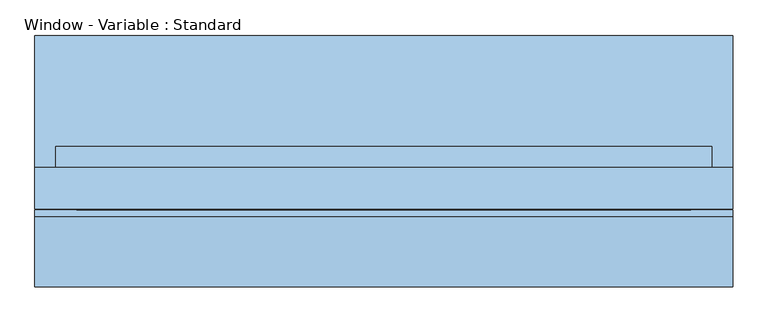
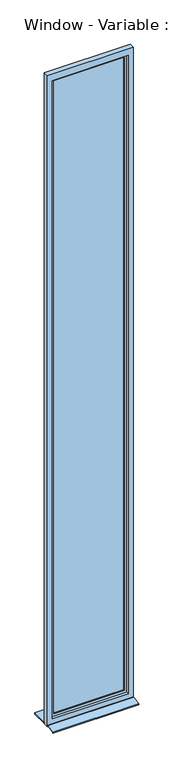
"""IFC4 building model written with IfcOpenShell, lengths in millimetres: window geometry, Window - Variable : Standard."""

import ifcopenshell
import ifcopenshell.guid

model = None  # the IFC model being written
_history = None  # IfcOwnerHistory: only IFC2X3 demands one
_inside = {}  # id of a spatial element -> (the spatial element, [elements in it])
_under = {}  # id of a project, library or spatial element -> (it, [spatial elements below it])
_declared = {}  # id of a project -> (the project, [libraries it declares])
_typed = {}  # id of a type object -> (the type object, [elements of that type])
_made_of = {}  # id of a material, layer set ... -> (it, [elements and type objects made of it])


def new_model(schema):
    """Start an empty IFC model of exactly this schema.

    Asked for "IFC4X3", IfcOpenShell would pick the latest addendum, in which some entities
    have other attributes; the version numbers below select the first issue.
    IFC2X3 requires an IfcOwnerHistory on every rooted entity: one is made here for all.
    """
    global model, _history
    if schema == "IFC4X3":
        model = ifcopenshell.file(schema_version=(4, 3, 0, 0))
    else:
        model = ifcopenshell.file(schema=schema)
    _inside.clear()
    _under.clear()
    _declared.clear()
    _typed.clear()
    _made_of.clear()
    _history = None
    if model.schema == "IFC2X3":
        org = make("IfcOrganization", Name="unknown")
        user = make(
            "IfcPersonAndOrganization",
            ThePerson=make("IfcPerson", FamilyName="unknown"),
            TheOrganization=org,
        )
        app = make(
            "IfcApplication",
            ApplicationDeveloper=org,
            Version="unknown",
            ApplicationFullName="unknown",
            ApplicationIdentifier="unknown",
        )
        _history = make(
            "IfcOwnerHistory",
            OwningUser=user,
            OwningApplication=app,
            ChangeAction="ADDED",
            CreationDate=0,
        )
    return model


def make(cls, **values):
    """One entity of the class cls with the attributes given. An attribute that is None is left unset."""
    return model.create_entity(
        cls, **{name: value for name, value in values.items() if value is not None}
    )


def rooted(cls, **values):
    """An entity with a GlobalId (a new one), such as an element, a storey or a relation."""
    return make(cls, GlobalId=ifcopenshell.guid.new(), OwnerHistory=_history, **values)


def si_unit(unit_type, name, prefix=None):
    """IfcSIUnit, for example si_unit("LENGTHUNIT", "METRE", prefix="MILLI")."""
    return make("IfcSIUnit", UnitType=unit_type, Prefix=prefix, Name=name)


def assignment(units):
    """IfcUnitAssignment: the units of a project."""
    return None if units is None else make("IfcUnitAssignment", Units=units)


def point(xyz):
    """IfcCartesianPoint."""
    return None if xyz is None else make("IfcCartesianPoint", Coordinates=xyz)


def direction(xyz):
    """IfcDirection."""
    return None if xyz is None else make("IfcDirection", DirectionRatios=xyz)


def frame(location, z_axis=None, x_axis=None):
    """IfcAxis2Placement3D, a coordinate frame: its origin and axes. An axis left out is left unset."""
    return make(
        "IfcAxis2Placement3D",
        Location=point(location),
        Axis=direction(z_axis),
        RefDirection=direction(x_axis),
    )


def origin():
    """The frame at (0, 0, 0) with its axes left unset."""
    return frame((0.0, 0.0, 0.0))


def place(relative_to, where):
    """IfcLocalPlacement: puts the frame where relative to a parent placement (None: the world)."""
    return make(
        "IfcLocalPlacement", PlacementRelTo=relative_to, RelativePlacement=where
    )


def context(
    kind, dimensions, precision=None, world=None, true_north=None, identifier=None
):
    """IfcGeometricRepresentationContext, for example the 3D "Model" context."""
    return make(
        "IfcGeometricRepresentationContext",
        ContextIdentifier=identifier,
        ContextType=kind,
        CoordinateSpaceDimension=dimensions,
        Precision=precision,
        WorldCoordinateSystem=world,
        TrueNorth=true_north,
    )


def project(units=None, contexts=None):
    """IfcProject with its units and contexts."""
    return rooted(
        "IfcProject",
        Name="project",
        RepresentationContexts=contexts,
        UnitsInContext=assignment(units),
    )


def spatial(cls, under=None, at=None, **own):
    """A site, building, storey or space (cls), placed at a placement, below another one or the project."""
    s = rooted(cls, ObjectPlacement=at, **own)
    if under is not None:
        _under.setdefault(under.id(), (under, []))[1].append(s)
    return s


def polyline(points):
    """IfcPolyline through the points."""
    return make("IfcPolyline", Points=[point(p) for p in points])


def outline(outer, holes=None, kind="AREA"):
    """IfcArbitraryClosedProfileDef: a profile drawn as a closed curve; with holes, ...WithVoids."""
    if holes is None:
        return make("IfcArbitraryClosedProfileDef", ProfileType=kind, OuterCurve=outer)
    return make(
        "IfcArbitraryProfileDefWithVoids",
        ProfileType=kind,
        OuterCurve=outer,
        InnerCurves=holes,
    )


def extrude(swept, where, along, depth):
    """IfcExtrudedAreaSolid: the profile swept, set in the frame where, extruded along a direction by depth."""
    return make(
        "IfcExtrudedAreaSolid",
        SweptArea=swept,
        Position=where,
        ExtrudedDirection=direction(along),
        Depth=depth,
    )


def faces_of(points, faces, orient=None, outer=None):
    """IfcFace entities. A face is a list of loops; a loop is a list of indices into points, from 0.

    orient and outer hold one flag for each loop. By default every Orientation is true, the
    first loop of a face is its IfcFaceOuterBound and the others are IfcFaceBound.
    """
    made = []
    for i, loops in enumerate(faces):
        bounds = []
        for j, loop in enumerate(loops):
            is_outer = j == 0 if outer is None else outer[i][j]
            bounds.append(
                make(
                    "IfcFaceOuterBound" if is_outer else "IfcFaceBound",
                    Bound=make("IfcPolyLoop", Polygon=[points[k] for k in loop]),
                    Orientation=True if orient is None else orient[i][j],
                )
            )
        made.append(make("IfcFace", Bounds=bounds))
    return made


def faceted_brep(points, faces, orient=None, outer=None, voids=None):
    """IfcFacetedBrep: a solid bounded by flat faces; with voids (closed shells), ...WithVoids."""
    shared = [point(p) for p in points]
    hull = make("IfcClosedShell", CfsFaces=faces_of(shared, faces, orient, outer))
    if voids is None:
        return make("IfcFacetedBrep", Outer=hull)
    return make(
        "IfcFacetedBrepWithVoids",
        Outer=hull,
        Voids=[
            make(cls, CfsFaces=faces_of(shared, fs, o, b)) for cls, fs, o, b in voids
        ],
    )


def shape(context_of_items, identifier, shape_type, items):
    """IfcShapeRepresentation: the items that make up one representation, for example the "Body"."""
    return make(
        "IfcShapeRepresentation",
        ContextOfItems=context_of_items,
        RepresentationIdentifier=identifier,
        RepresentationType=shape_type,
        Items=items,
    )


def source(mapping_origin, context_of_items, identifier, shape_type, items):
    """IfcRepresentationMap: a shape defined once, which mapped items show again and again."""
    return make(
        "IfcRepresentationMap",
        MappingOrigin=mapping_origin,
        MappedRepresentation=shape(context_of_items, identifier, shape_type, items),
    )


def transform(
    local_origin,
    x_axis=None,
    y_axis=None,
    z_axis=None,
    scale=None,
    scale2=None,
    scale3=None,
    uniform=True,
):
    """IfcCartesianTransformationOperator3D, or its non-uniform kind. x_axis, y_axis, z_axis: its Axis1, 2, 3."""
    if uniform:
        return make(
            "IfcCartesianTransformationOperator3D",
            Axis1=direction(x_axis),
            Axis2=direction(y_axis),
            LocalOrigin=point(local_origin),
            Scale=scale,
            Axis3=direction(z_axis),
        )
    return make(
        "IfcCartesianTransformationOperator3DnonUniform",
        Axis1=direction(x_axis),
        Axis2=direction(y_axis),
        LocalOrigin=point(local_origin),
        Scale=scale,
        Axis3=direction(z_axis),
        Scale2=scale2,
        Scale3=scale3,
    )


def mapped(mapping_source, mapping_target):
    """IfcMappedItem: shows the shape of a source again, moved by a transform."""
    return make(
        "IfcMappedItem", MappingSource=mapping_source, MappingTarget=mapping_target
    )


def made_of(thing, what):
    """Note that an element or type object is made of a material, layer set ...; save() writes the relation."""
    if what is not None:
        _made_of.setdefault(what.id(), (what, []))[1].append(thing)
    return thing


def element(
    cls,
    number,
    at=None,
    inside=None,
    cuts=None,
    type_object=None,
    material=None,
    context=None,
    identifier="Body",
    shape_type=None,
    held_by="IfcProductDefinitionShape",
    body=None,
    shapes=None,
    **own,
):
    """One element of the class cls, such as IfcWall. Its Tag is "e" and its number.

    at: its placement. inside: the storey or other place that contains it. cuts: it is an
    opening in that element (IfcRelVoidsElement). A single representation is given by context,
    identifier, shape_type and body (its items); several are given by shapes. held_by: the class
    of the entity that holds the representations. save() writes the other relations.
    """
    e = rooted(cls, Tag="e%d" % number, ObjectPlacement=at, **own)
    if body is not None:
        shapes = [shape(context, identifier, shape_type, body)]
    if shapes is not None:
        e.Representation = make(held_by, Representations=shapes)
    if inside is not None:
        _inside.setdefault(inside.id(), (inside, []))[1].append(e)
    if cuts is not None:
        rooted(
            "IfcRelVoidsElement", RelatingBuildingElement=cuts, RelatedOpeningElement=e
        )
    if type_object is not None:
        _typed.setdefault(type_object.id(), (type_object, []))[1].append(e)
    return made_of(e, material)


def aggregate(whole, parts):
    """IfcRelAggregates: a whole, such as a stair, and the parts it consists of."""
    return rooted("IfcRelAggregates", RelatingObject=whole, RelatedObjects=parts)


def save(model, path):
    """Write the relations noted so far, then the file.

    IfcRelAggregates (storeys below a building ...), IfcRelContainedInSpatialStructure (elements
    in a storey), IfcRelDefinesByType, IfcRelAssociatesMaterial and IfcRelDeclares: one each for
    every whole, place, type object, material and project.
    """
    for whole, parts in _under.values():
        aggregate(whole, parts)
    for where, things in _inside.values():
        rooted(
            "IfcRelContainedInSpatialStructure",
            RelatedElements=things,
            RelatingStructure=where,
        )
    for kind, things in _typed.values():
        rooted("IfcRelDefinesByType", RelatedObjects=things, RelatingType=kind)
    for what, things in _made_of.values():
        rooted("IfcRelAssociatesMaterial", RelatedObjects=things, RelatingMaterial=what)
    for by, libraries in _declared.values():
        rooted("IfcRelDeclares", RelatingContext=by, RelatedDefinitions=libraries)
    model.write(path)


def window_variable_standard_9eb8f332(model_context):
    return source(origin(), model_context, "Body", "SolidModel", [
        extrude(outline(polyline([(9000.0, 500.0), (9000.0, -500.0), (1000.0, -500.0), (1000.0, 500.0), (9000.0, 500.0)]), holes=[polyline([(8920.0, 440.0), (1080.0, 440.0), (1080.0, -440.0), (8920.0, -440.0), (8920.0, 440.0)])]), frame((0.0, -70.0, 0.0), z_axis=(0.0, 1.0, 0.0), x_axis=(0.0, 0.0, 1.0)), (0.0, 0.0, 1.0), 60.0),
        faceted_brep([(470.0, -10.0, 8950.0), (470.0, -10.0, 1050.0), (470.0, 20.0, 1050.0), (470.0, 20.0, 8950.0), (-470.0, 20.0, 1050.0), (-470.0, 20.0, 8950.0), (410.0, 20.0, 1110.0), (410.0, 20.0, 8890.0), (-410.0, 20.0, 8890.0), (-410.0, 20.0, 1110.0), (-470.0, -10.0, 1050.0), (-470.0, -10.0, 8950.0), (440.0, -10.0, 8920.0), (440.0, -10.0, 1080.0), (-440.0, -10.0, 1080.0), (-440.0, -10.0, 8920.0), (440.0, -40.0, 8920.0), (440.0, -40.0, 1080.0), (-440.0, -40.0, 1080.0), (-440.0, -40.0, 8920.0), (410.0, -40.0, 8890.0), (410.0, -40.0, 1110.0), (-410.0, -40.0, 1110.0), (-410.0, -40.0, 8890.0)], [[[0, 1, 2, 3]], [[3, 2, 4, 5], [6, 7, 8, 9]], [[1, 10, 4, 2]], [[1, 0, 11, 10], [12, 13, 14, 15]], [[16, 17, 13, 12]], [[17, 18, 14, 13]], [[17, 16, 19, 18], [20, 21, 22, 23]], [[7, 6, 21, 20]], [[6, 9, 22, 21]], [[10, 11, 5, 4]], [[18, 19, 15, 14]], [[9, 8, 23, 22]], [[11, 0, 3, 5]], [[19, 16, 12, 15]], [[8, 7, 20, 23]]]),
        extrude(outline(polyline([(-500.0, 180.0), (500.0, 180.0), (500.0, -10.0), (-500.0, -10.0), (-500.0, 180.0)])), frame((0.0, 0.0, 1005.0), z_axis=(0.0, 0.0, 1.0), x_axis=(1.0, 0.0, 0.0)), (0.0, 0.0, 1.0), 15.0),
        extrude(outline(polyline([(-80.0221543, 1020.0), (-70.0, 1020.0), (-70.0, 1018.0), (-79.8240723, 1018.0), (-178.0, 998.3604634), (-178.0, 990.0), (-180.0, 990.0), (-180.0, 1000.0), (-80.0221543, 1020.0)])), frame((-500.0, 0.0, 0.0), z_axis=(1.0, 0.0, 0.0), x_axis=(0.0, 1.0, 0.0)), (0.0, 0.0, 1.0), 1000.0),
        extrude(outline(polyline([(410.0, 5.0), (410.0, -25.0), (-410.0, -25.0), (-410.0, 5.0), (410.0, 5.0)])), frame((0.0, 0.0, 1110.0), z_axis=(0.0, 0.0, 1.0), x_axis=(1.0, 0.0, 0.0)), (0.0, 0.0, 1.0), 7780.0),
    ])


if __name__ == "__main__":
    model = new_model("IFC4")
    model_context = context("Model", 3, world=origin())
    ifc_project = project(units=[si_unit("LENGTHUNIT", "METRE", prefix="MILLI")], contexts=[model_context])
    site = spatial("IfcSite", under=ifc_project)
    building = spatial("IfcBuilding", under=site)
    placement = place(None, origin())
    window_variable_standard_shape = window_variable_standard_9eb8f332(model_context)
    element("IfcWindow", 1, ObjectType="Window - Variable : Standard", at=placement, inside=building, context=model_context, shape_type="MappedRepresentation", body=[
        mapped(window_variable_standard_shape, transform((0.0, 0.0, 0.0), x_axis=(1.0, 0.0, 0.0), y_axis=(0.0, 1.0, 0.0), z_axis=(0.0, 0.0, 1.0))),
    ])
    save(model, "model.ifc")

# Revit data of these elements
# Type "Window - Variable : Standard"
#   Type Mark = "19"
#   Operation = "SinglePanel"
#   Keynote = "16.05.01"
#   Analytic Construction = "<None>"
#   Rough Width [instance default] = 1.010 m
#   Rough Height [instance default] = 1.010 m
#   Frame Depth = 0.060 m
#   Frame Height Bottom = 0.080 m
#   Frame Height Top = 0.080 m
#   Frame Width = 0.060 m
#   Height [instance default] = 1.010 m
#   Window Inset = 0.060 m
#   Window Width = 0.060 m
#   Instalation Depth [instance default] = 0.080 m
#   Width [instance default] = 1.010 m
#   Folding Wing [instance default] = no
#   Oppening Direction Vertical [instance default] = yes
#   Oppening Direction Visibility [instance default] = no
#   Casement [instance default] = yes
#   Frame [instance default] = none
#   Glas [instance default] = none
#   Window [instance default] = none
#   Windowsill Inside [instance default] = none
#   Windowsill Outside [instance default] = none
#   Wall Closure = (empty or 0)
#   Assembly Code = ""
# Element 1 (IfcWindow, "Window - Variable : Standard")
#   Rough Width = 1.000 m
#   Rough Height = 8.000 m
#   Height = 8.000 m
#   Width = 1.000 m
#   Materials on its faces: "Plastic - White", "Metal _ Aluminium", "Wood - Birch", "Glass"
# Materials
#   "Plastic - White": class "Kunststoff", colour RGB 249 249 249, transparency 0
#   "Metal _ Aluminium": class "Metall", colour RGB 247 247 247, transparency 0
#   "Wood - Birch": class "Holz", colour RGB 213 164 103, transparency 0
#   "Glass": class "Glass", colour RGB 0 128 192, transparency 0.9
